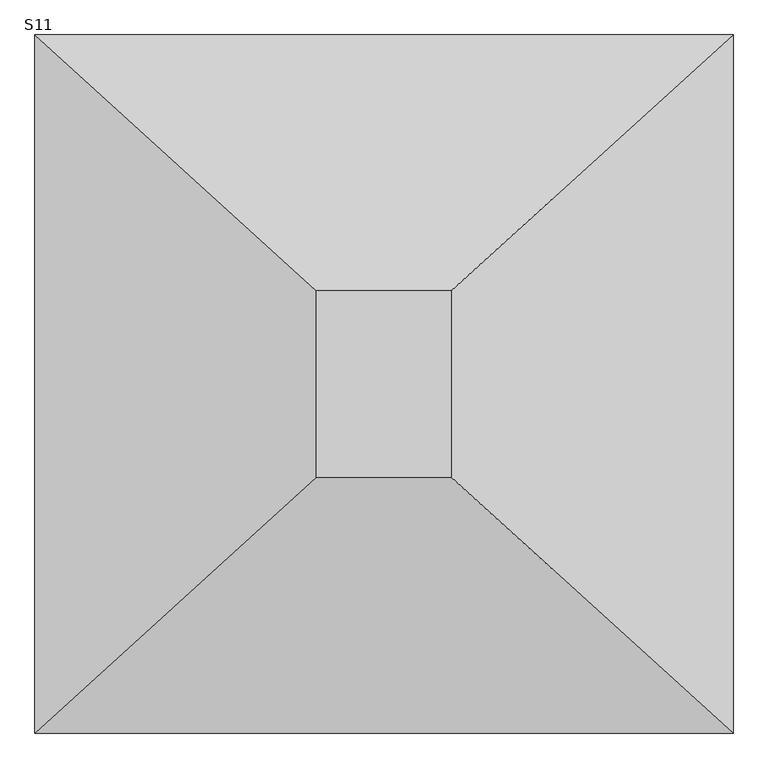
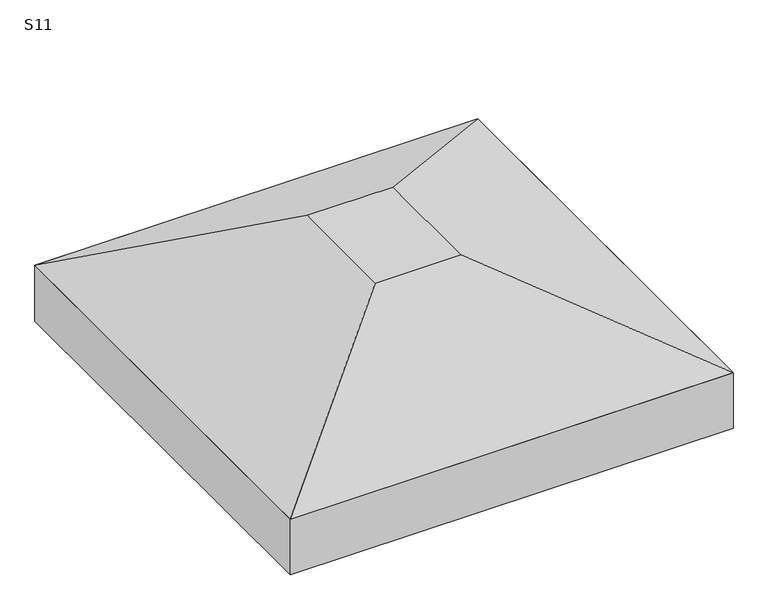
"""IFC4 building model written with IfcOpenShell, lengths in millimetres: fastener geometry, TQS - Sapata : S11."""

from ifc_helpers import new_model, si_unit, frame, origin, place, context, project, spatial, polyline, outline, extrude, faceted_brep, source, transform, mapped, element, save


def s11_36e66e76(model_context):
    return source(origin(), model_context, "Body", "SolidModel", [
        faceted_brep([(-55.0, 0.0, 0.0), (-345.0, 0.0, 0.0), (-345.0, -400.0, 0.0), (-55.0, -400.0, 0.0), (550.0, 550.0, -300.0), (550.0, -950.0, -300.0), (-950.0, -950.0, -300.0), (-950.0, 550.0, -300.0)], [[[0, 1, 2, 3]], [[4, 5, 6, 7]], [[4, 7, 1, 0]], [[7, 6, 2, 1]], [[6, 5, 3, 2]], [[5, 4, 0, 3]]]),
        extrude(outline(polyline([(550.0, 550.0), (550.0, -950.0), (-950.0, -950.0), (-950.0, 550.0), (550.0, 550.0)])), frame((0.0, 0.0, -500.0), z_axis=(0.0, 0.0, 1.0), x_axis=(1.0, 0.0, 0.0)), (0.0, 0.0, 1.0), 200.0),
    ])


if __name__ == "__main__":
    model = new_model("IFC4")
    model_context = context("Model", 3, world=origin())
    ifc_project = project(units=[si_unit("LENGTHUNIT", "METRE", prefix="MILLI")], contexts=[model_context])
    site = spatial("IfcSite", under=ifc_project)
    building = spatial("IfcBuilding", under=site)
    placement = place(None, origin())
    s11_shape = s11_36e66e76(model_context)
    element("IfcFastener", 1, ObjectType="TQS - Sapata : S11", at=placement, inside=building, context=model_context, shape_type="MappedRepresentation", body=[
        mapped(s11_shape, transform((0.0, 0.0, 0.0), x_axis=(1.0, 0.0, 0.0), y_axis=(0.0, 1.0, 0.0), z_axis=(0.0, 0.0, 1.0))),
    ])
    save(model, "model.ifc")

# Revit data of these elements
# Type "TQS - Sapata : S11"
#   TY = 0.40 m
#   TX = 0.29 m
#   HS = 0.50 m
#   H0 = 0.20 m
#   EXCYABS = 0.75 m
#   EXCY = 0.00 m
#   EXCXABS = 0.75 m
#   EXCX = 0.00 m
#   DIMY = 1.50 m
#   DIMX = 1.50 m
#   Material estrutural = Concreto - Concreto concretado no local
#   Width = 0
#   Length = 0
# Element 1 (IfcFastener, "TQS - Sapata : S11")
#   Materials on its faces: "Concreto - Concreto concretado no local"
# Materials
#   "Concreto - Concreto concretado no local": class "Concreto", colour RGB 192 192 192, transparency 0
